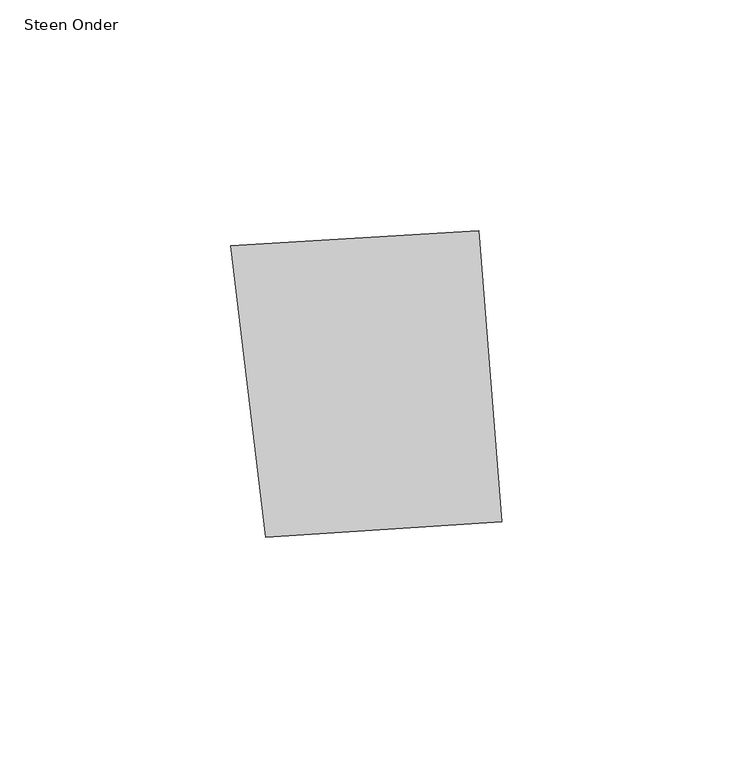
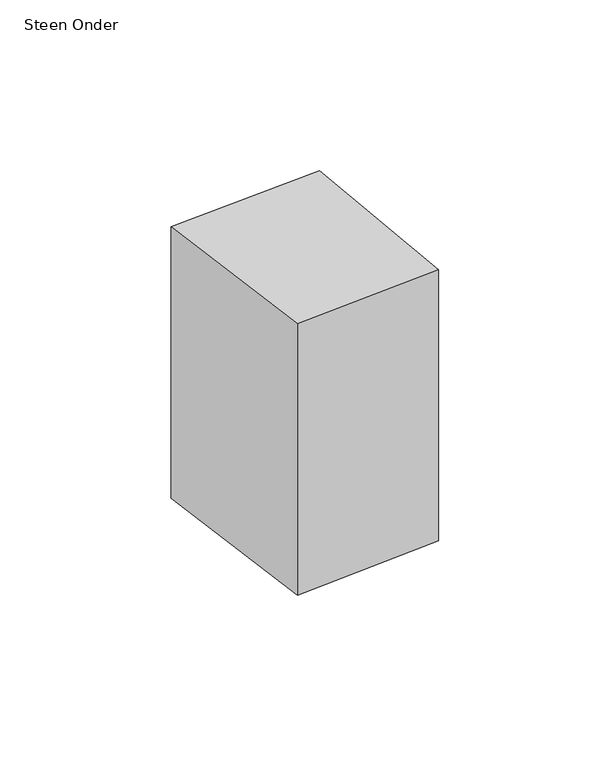
"""IFC4 building model written with IfcOpenShell, lengths in millimetres: proxy geometry, 00_GMA_steen_versie_4 : Steen Onder."""

import ifcopenshell
import ifcopenshell.guid

model = None  # the IFC model being written
_history = None  # IfcOwnerHistory: only IFC2X3 demands one
_inside = {}  # id of a spatial element -> (the spatial element, [elements in it])
_under = {}  # id of a project, library or spatial element -> (it, [spatial elements below it])
_declared = {}  # id of a project -> (the project, [libraries it declares])
_typed = {}  # id of a type object -> (the type object, [elements of that type])
_made_of = {}  # id of a material, layer set ... -> (it, [elements and type objects made of it])


def new_model(schema):
    """Start an empty IFC model of exactly this schema.

    Asked for "IFC4X3", IfcOpenShell would pick the latest addendum, in which some entities
    have other attributes; the version numbers below select the first issue.
    IFC2X3 requires an IfcOwnerHistory on every rooted entity: one is made here for all.
    """
    global model, _history
    if schema == "IFC4X3":
        model = ifcopenshell.file(schema_version=(4, 3, 0, 0))
    else:
        model = ifcopenshell.file(schema=schema)
    _inside.clear()
    _under.clear()
    _declared.clear()
    _typed.clear()
    _made_of.clear()
    _history = None
    if model.schema == "IFC2X3":
        org = make("IfcOrganization", Name="unknown")
        user = make(
            "IfcPersonAndOrganization",
            ThePerson=make("IfcPerson", FamilyName="unknown"),
            TheOrganization=org,
        )
        app = make(
            "IfcApplication",
            ApplicationDeveloper=org,
            Version="unknown",
            ApplicationFullName="unknown",
            ApplicationIdentifier="unknown",
        )
        _history = make(
            "IfcOwnerHistory",
            OwningUser=user,
            OwningApplication=app,
            ChangeAction="ADDED",
            CreationDate=0,
        )
    return model


def make(cls, **values):
    """One entity of the class cls with the attributes given. An attribute that is None is left unset."""
    return model.create_entity(
        cls, **{name: value for name, value in values.items() if value is not None}
    )


def rooted(cls, **values):
    """An entity with a GlobalId (a new one), such as an element, a storey or a relation."""
    return make(cls, GlobalId=ifcopenshell.guid.new(), OwnerHistory=_history, **values)


def si_unit(unit_type, name, prefix=None):
    """IfcSIUnit, for example si_unit("LENGTHUNIT", "METRE", prefix="MILLI")."""
    return make("IfcSIUnit", UnitType=unit_type, Prefix=prefix, Name=name)


def assignment(units):
    """IfcUnitAssignment: the units of a project."""
    return None if units is None else make("IfcUnitAssignment", Units=units)


def point(xyz):
    """IfcCartesianPoint."""
    return None if xyz is None else make("IfcCartesianPoint", Coordinates=xyz)


def direction(xyz):
    """IfcDirection."""
    return None if xyz is None else make("IfcDirection", DirectionRatios=xyz)


def frame(location, z_axis=None, x_axis=None):
    """IfcAxis2Placement3D, a coordinate frame: its origin and axes. An axis left out is left unset."""
    return make(
        "IfcAxis2Placement3D",
        Location=point(location),
        Axis=direction(z_axis),
        RefDirection=direction(x_axis),
    )


def origin():
    """The frame at (0, 0, 0) with its axes left unset."""
    return frame((0.0, 0.0, 0.0))


def origin_with_axes():
    """The frame at (0, 0, 0) with the z axis (0, 0, 1) and the x axis (1, 0, 0) written out."""
    return frame((0.0, 0.0, 0.0), z_axis=(0.0, 0.0, 1.0), x_axis=(1.0, 0.0, 0.0))


def place(relative_to, where):
    """IfcLocalPlacement: puts the frame where relative to a parent placement (None: the world)."""
    return make(
        "IfcLocalPlacement", PlacementRelTo=relative_to, RelativePlacement=where
    )


def context(
    kind, dimensions, precision=None, world=None, true_north=None, identifier=None
):
    """IfcGeometricRepresentationContext, for example the 3D "Model" context."""
    return make(
        "IfcGeometricRepresentationContext",
        ContextIdentifier=identifier,
        ContextType=kind,
        CoordinateSpaceDimension=dimensions,
        Precision=precision,
        WorldCoordinateSystem=world,
        TrueNorth=true_north,
    )


def project(units=None, contexts=None):
    """IfcProject with its units and contexts."""
    return rooted(
        "IfcProject",
        Name="project",
        RepresentationContexts=contexts,
        UnitsInContext=assignment(units),
    )


def spatial(cls, under=None, at=None, **own):
    """A site, building, storey or space (cls), placed at a placement, below another one or the project."""
    s = rooted(cls, ObjectPlacement=at, **own)
    if under is not None:
        _under.setdefault(under.id(), (under, []))[1].append(s)
    return s


def polyline(points):
    """IfcPolyline through the points."""
    return make("IfcPolyline", Points=[point(p) for p in points])


def outline(outer, holes=None, kind="AREA"):
    """IfcArbitraryClosedProfileDef: a profile drawn as a closed curve; with holes, ...WithVoids."""
    if holes is None:
        return make("IfcArbitraryClosedProfileDef", ProfileType=kind, OuterCurve=outer)
    return make(
        "IfcArbitraryProfileDefWithVoids",
        ProfileType=kind,
        OuterCurve=outer,
        InnerCurves=holes,
    )


def extrude(swept, where, along, depth):
    """IfcExtrudedAreaSolid: the profile swept, set in the frame where, extruded along a direction by depth."""
    return make(
        "IfcExtrudedAreaSolid",
        SweptArea=swept,
        Position=where,
        ExtrudedDirection=direction(along),
        Depth=depth,
    )


def shape(context_of_items, identifier, shape_type, items):
    """IfcShapeRepresentation: the items that make up one representation, for example the "Body"."""
    return make(
        "IfcShapeRepresentation",
        ContextOfItems=context_of_items,
        RepresentationIdentifier=identifier,
        RepresentationType=shape_type,
        Items=items,
    )


def source(mapping_origin, context_of_items, identifier, shape_type, items):
    """IfcRepresentationMap: a shape defined once, which mapped items show again and again."""
    return make(
        "IfcRepresentationMap",
        MappingOrigin=mapping_origin,
        MappedRepresentation=shape(context_of_items, identifier, shape_type, items),
    )


def transform(
    local_origin,
    x_axis=None,
    y_axis=None,
    z_axis=None,
    scale=None,
    scale2=None,
    scale3=None,
    uniform=True,
):
    """IfcCartesianTransformationOperator3D, or its non-uniform kind. x_axis, y_axis, z_axis: its Axis1, 2, 3."""
    if uniform:
        return make(
            "IfcCartesianTransformationOperator3D",
            Axis1=direction(x_axis),
            Axis2=direction(y_axis),
            LocalOrigin=point(local_origin),
            Scale=scale,
            Axis3=direction(z_axis),
        )
    return make(
        "IfcCartesianTransformationOperator3DnonUniform",
        Axis1=direction(x_axis),
        Axis2=direction(y_axis),
        LocalOrigin=point(local_origin),
        Scale=scale,
        Axis3=direction(z_axis),
        Scale2=scale2,
        Scale3=scale3,
    )


def mapped(mapping_source, mapping_target):
    """IfcMappedItem: shows the shape of a source again, moved by a transform."""
    return make(
        "IfcMappedItem", MappingSource=mapping_source, MappingTarget=mapping_target
    )


def made_of(thing, what):
    """Note that an element or type object is made of a material, layer set ...; save() writes the relation."""
    if what is not None:
        _made_of.setdefault(what.id(), (what, []))[1].append(thing)
    return thing


def element(
    cls,
    number,
    at=None,
    inside=None,
    cuts=None,
    type_object=None,
    material=None,
    context=None,
    identifier="Body",
    shape_type=None,
    held_by="IfcProductDefinitionShape",
    body=None,
    shapes=None,
    **own,
):
    """One element of the class cls, such as IfcWall. Its Tag is "e" and its number.

    at: its placement. inside: the storey or other place that contains it. cuts: it is an
    opening in that element (IfcRelVoidsElement). A single representation is given by context,
    identifier, shape_type and body (its items); several are given by shapes. held_by: the class
    of the entity that holds the representations. save() writes the other relations.
    """
    e = rooted(cls, Tag="e%d" % number, ObjectPlacement=at, **own)
    if body is not None:
        shapes = [shape(context, identifier, shape_type, body)]
    if shapes is not None:
        e.Representation = make(held_by, Representations=shapes)
    if inside is not None:
        _inside.setdefault(inside.id(), (inside, []))[1].append(e)
    if cuts is not None:
        rooted(
            "IfcRelVoidsElement", RelatingBuildingElement=cuts, RelatedOpeningElement=e
        )
    if type_object is not None:
        _typed.setdefault(type_object.id(), (type_object, []))[1].append(e)
    return made_of(e, material)


def aggregate(whole, parts):
    """IfcRelAggregates: a whole, such as a stair, and the parts it consists of."""
    return rooted("IfcRelAggregates", RelatingObject=whole, RelatedObjects=parts)


def save(model, path):
    """Write the relations noted so far, then the file.

    IfcRelAggregates (storeys below a building ...), IfcRelContainedInSpatialStructure (elements
    in a storey), IfcRelDefinesByType, IfcRelAssociatesMaterial and IfcRelDeclares: one each for
    every whole, place, type object, material and project.
    """
    for whole, parts in _under.values():
        aggregate(whole, parts)
    for where, things in _inside.values():
        rooted(
            "IfcRelContainedInSpatialStructure",
            RelatedElements=things,
            RelatingStructure=where,
        )
    for kind, things in _typed.values():
        rooted("IfcRelDefinesByType", RelatedObjects=things, RelatingType=kind)
    for what, things in _made_of.values():
        rooted("IfcRelAssociatesMaterial", RelatedObjects=things, RelatingMaterial=what)
    for by, libraries in _declared.values():
        rooted("IfcRelDeclares", RelatingContext=by, RelatedDefinitions=libraries)
    model.write(path)


def steen_onder_aafd55e8(model_context):
    return source(origin(), model_context, "Body", "SweptSolid", [
        extrude(outline(polyline([(98.2243602, 97.3820858), (103.2960473, 34.2995155), (52.1118821, 30.9502314), (44.518619, 94.1404935), (98.2243602, 97.3820858)])), origin_with_axes(), (0.0, 0.0, 1.0), 100.0),
    ])


if __name__ == "__main__":
    model = new_model("IFC4")
    model_context = context("Model", 3, world=origin())
    ifc_project = project(units=[si_unit("LENGTHUNIT", "METRE", prefix="MILLI")], contexts=[model_context])
    site = spatial("IfcSite", under=ifc_project)
    building = spatial("IfcBuilding", under=site)
    placement = place(None, origin())
    steen_onder_shape = steen_onder_aafd55e8(model_context)
    element("IfcBuildingElementProxy", 1, Name="00_GMA_steen_versie_4 : Steen Onder", ObjectType="00_GMA_steen_versie_4 : Steen Onder", at=placement, inside=building, context=model_context, shape_type="MappedRepresentation", body=[
        mapped(steen_onder_shape, transform((0.0, 0.0, 0.0), x_axis=(1.0, 0.0, 0.0), y_axis=(0.0, 1.0, 0.0), z_axis=(0.0, 0.0, 1.0))),
    ])
    save(model, "model.ifc")

# Revit data of these elements
# Type "00_GMA_steen_versie_4 : Steen Onder"
#   StootVoegHalfBoven [instance default] = 5 mm
#   StootVoegHalf [instance default] = 5 mm
#   StootVoegBreedteOnder = 10 mm
#   StootVoegBreedteBoven = 10 mm
#   Steendikte = 100 mm
#   LintVoegOnderHalf = 0 mm
#   LintVoegOnder = 0 mm
#   LintVoegBovenHalf = 5 mm
#   LintVoegBoven = 10 mm
#   materiaal = none
#   MateriaalVoeg = none
#   Default Elevation = 0
